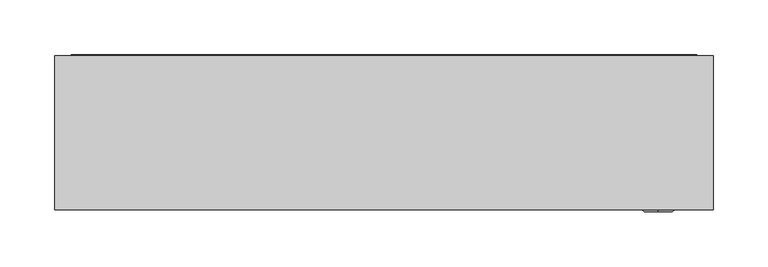
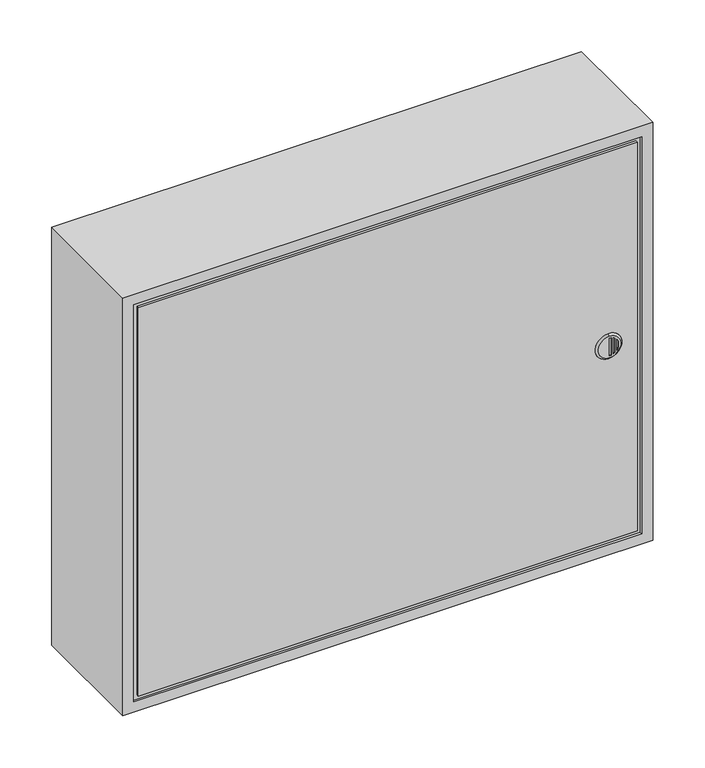
"""IFC4 building model written with IfcOpenShell, lengths in millimetres: proxy geometry, Unterverteiler : groß AP (120 PLE)."""

import ifcopenshell
import ifcopenshell.guid

model = None  # the IFC model being written
_history = None  # IfcOwnerHistory: only IFC2X3 demands one
_inside = {}  # id of a spatial element -> (the spatial element, [elements in it])
_under = {}  # id of a project, library or spatial element -> (it, [spatial elements below it])
_declared = {}  # id of a project -> (the project, [libraries it declares])
_typed = {}  # id of a type object -> (the type object, [elements of that type])
_made_of = {}  # id of a material, layer set ... -> (it, [elements and type objects made of it])


def new_model(schema):
    """Start an empty IFC model of exactly this schema.

    Asked for "IFC4X3", IfcOpenShell would pick the latest addendum, in which some entities
    have other attributes; the version numbers below select the first issue.
    IFC2X3 requires an IfcOwnerHistory on every rooted entity: one is made here for all.
    """
    global model, _history
    if schema == "IFC4X3":
        model = ifcopenshell.file(schema_version=(4, 3, 0, 0))
    else:
        model = ifcopenshell.file(schema=schema)
    _inside.clear()
    _under.clear()
    _declared.clear()
    _typed.clear()
    _made_of.clear()
    _history = None
    if model.schema == "IFC2X3":
        org = make("IfcOrganization", Name="unknown")
        user = make(
            "IfcPersonAndOrganization",
            ThePerson=make("IfcPerson", FamilyName="unknown"),
            TheOrganization=org,
        )
        app = make(
            "IfcApplication",
            ApplicationDeveloper=org,
            Version="unknown",
            ApplicationFullName="unknown",
            ApplicationIdentifier="unknown",
        )
        _history = make(
            "IfcOwnerHistory",
            OwningUser=user,
            OwningApplication=app,
            ChangeAction="ADDED",
            CreationDate=0,
        )
    return model


def make(cls, **values):
    """One entity of the class cls with the attributes given. An attribute that is None is left unset."""
    return model.create_entity(
        cls, **{name: value for name, value in values.items() if value is not None}
    )


def rooted(cls, **values):
    """An entity with a GlobalId (a new one), such as an element, a storey or a relation."""
    return make(cls, GlobalId=ifcopenshell.guid.new(), OwnerHistory=_history, **values)


def si_unit(unit_type, name, prefix=None):
    """IfcSIUnit, for example si_unit("LENGTHUNIT", "METRE", prefix="MILLI")."""
    return make("IfcSIUnit", UnitType=unit_type, Prefix=prefix, Name=name)


def assignment(units):
    """IfcUnitAssignment: the units of a project."""
    return None if units is None else make("IfcUnitAssignment", Units=units)


def point(xyz):
    """IfcCartesianPoint."""
    return None if xyz is None else make("IfcCartesianPoint", Coordinates=xyz)


def direction(xyz):
    """IfcDirection."""
    return None if xyz is None else make("IfcDirection", DirectionRatios=xyz)


def frame(location, z_axis=None, x_axis=None):
    """IfcAxis2Placement3D, a coordinate frame: its origin and axes. An axis left out is left unset."""
    return make(
        "IfcAxis2Placement3D",
        Location=point(location),
        Axis=direction(z_axis),
        RefDirection=direction(x_axis),
    )


def origin():
    """The frame at (0, 0, 0) with its axes left unset."""
    return frame((0.0, 0.0, 0.0))


def place(relative_to, where):
    """IfcLocalPlacement: puts the frame where relative to a parent placement (None: the world)."""
    return make(
        "IfcLocalPlacement", PlacementRelTo=relative_to, RelativePlacement=where
    )


def context(
    kind, dimensions, precision=None, world=None, true_north=None, identifier=None
):
    """IfcGeometricRepresentationContext, for example the 3D "Model" context."""
    return make(
        "IfcGeometricRepresentationContext",
        ContextIdentifier=identifier,
        ContextType=kind,
        CoordinateSpaceDimension=dimensions,
        Precision=precision,
        WorldCoordinateSystem=world,
        TrueNorth=true_north,
    )


def project(units=None, contexts=None):
    """IfcProject with its units and contexts."""
    return rooted(
        "IfcProject",
        Name="project",
        RepresentationContexts=contexts,
        UnitsInContext=assignment(units),
    )


def spatial(cls, under=None, at=None, **own):
    """A site, building, storey or space (cls), placed at a placement, below another one or the project."""
    s = rooted(cls, ObjectPlacement=at, **own)
    if under is not None:
        _under.setdefault(under.id(), (under, []))[1].append(s)
    return s


def polyline(points):
    """IfcPolyline through the points."""
    return make("IfcPolyline", Points=[point(p) for p in points])


def circle_curve(where, radius):
    """IfcCircle in the frame where."""
    return make("IfcCircle", Position=where, Radius=radius)


def outline(outer, holes=None, kind="AREA"):
    """IfcArbitraryClosedProfileDef: a profile drawn as a closed curve; with holes, ...WithVoids."""
    if holes is None:
        return make("IfcArbitraryClosedProfileDef", ProfileType=kind, OuterCurve=outer)
    return make(
        "IfcArbitraryProfileDefWithVoids",
        ProfileType=kind,
        OuterCurve=outer,
        InnerCurves=holes,
    )


def extrude(swept, where, along, depth):
    """IfcExtrudedAreaSolid: the profile swept, set in the frame where, extruded along a direction by depth."""
    return make(
        "IfcExtrudedAreaSolid",
        SweptArea=swept,
        Position=where,
        ExtrudedDirection=direction(along),
        Depth=depth,
    )


def shape(context_of_items, identifier, shape_type, items):
    """IfcShapeRepresentation: the items that make up one representation, for example the "Body"."""
    return make(
        "IfcShapeRepresentation",
        ContextOfItems=context_of_items,
        RepresentationIdentifier=identifier,
        RepresentationType=shape_type,
        Items=items,
    )


def source(mapping_origin, context_of_items, identifier, shape_type, items):
    """IfcRepresentationMap: a shape defined once, which mapped items show again and again."""
    return make(
        "IfcRepresentationMap",
        MappingOrigin=mapping_origin,
        MappedRepresentation=shape(context_of_items, identifier, shape_type, items),
    )


def transform(
    local_origin,
    x_axis=None,
    y_axis=None,
    z_axis=None,
    scale=None,
    scale2=None,
    scale3=None,
    uniform=True,
):
    """IfcCartesianTransformationOperator3D, or its non-uniform kind. x_axis, y_axis, z_axis: its Axis1, 2, 3."""
    if uniform:
        return make(
            "IfcCartesianTransformationOperator3D",
            Axis1=direction(x_axis),
            Axis2=direction(y_axis),
            LocalOrigin=point(local_origin),
            Scale=scale,
            Axis3=direction(z_axis),
        )
    return make(
        "IfcCartesianTransformationOperator3DnonUniform",
        Axis1=direction(x_axis),
        Axis2=direction(y_axis),
        LocalOrigin=point(local_origin),
        Scale=scale,
        Axis3=direction(z_axis),
        Scale2=scale2,
        Scale3=scale3,
    )


def mapped(mapping_source, mapping_target):
    """IfcMappedItem: shows the shape of a source again, moved by a transform."""
    return make(
        "IfcMappedItem", MappingSource=mapping_source, MappingTarget=mapping_target
    )


def made_of(thing, what):
    """Note that an element or type object is made of a material, layer set ...; save() writes the relation."""
    if what is not None:
        _made_of.setdefault(what.id(), (what, []))[1].append(thing)
    return thing


def element(
    cls,
    number,
    at=None,
    inside=None,
    cuts=None,
    type_object=None,
    material=None,
    context=None,
    identifier="Body",
    shape_type=None,
    held_by="IfcProductDefinitionShape",
    body=None,
    shapes=None,
    **own,
):
    """One element of the class cls, such as IfcWall. Its Tag is "e" and its number.

    at: its placement. inside: the storey or other place that contains it. cuts: it is an
    opening in that element (IfcRelVoidsElement). A single representation is given by context,
    identifier, shape_type and body (its items); several are given by shapes. held_by: the class
    of the entity that holds the representations. save() writes the other relations.
    """
    e = rooted(cls, Tag="e%d" % number, ObjectPlacement=at, **own)
    if body is not None:
        shapes = [shape(context, identifier, shape_type, body)]
    if shapes is not None:
        e.Representation = make(held_by, Representations=shapes)
    if inside is not None:
        _inside.setdefault(inside.id(), (inside, []))[1].append(e)
    if cuts is not None:
        rooted(
            "IfcRelVoidsElement", RelatingBuildingElement=cuts, RelatedOpeningElement=e
        )
    if type_object is not None:
        _typed.setdefault(type_object.id(), (type_object, []))[1].append(e)
    return made_of(e, material)


def aggregate(whole, parts):
    """IfcRelAggregates: a whole, such as a stair, and the parts it consists of."""
    return rooted("IfcRelAggregates", RelatingObject=whole, RelatedObjects=parts)


def save(model, path):
    """Write the relations noted so far, then the file.

    IfcRelAggregates (storeys below a building ...), IfcRelContainedInSpatialStructure (elements
    in a storey), IfcRelDefinesByType, IfcRelAssociatesMaterial and IfcRelDeclares: one each for
    every whole, place, type object, material and project.
    """
    for whole, parts in _under.values():
        aggregate(whole, parts)
    for where, things in _inside.values():
        rooted(
            "IfcRelContainedInSpatialStructure",
            RelatedElements=things,
            RelatingStructure=where,
        )
    for kind, things in _typed.values():
        rooted("IfcRelDefinesByType", RelatedObjects=things, RelatingType=kind)
    for what, things in _made_of.values():
        rooted("IfcRelAssociatesMaterial", RelatedObjects=things, RelatingMaterial=what)
    for by, libraries in _declared.values():
        rooted("IfcRelDeclares", RelatingContext=by, RelatedDefinitions=libraries)
    model.write(path)


def plane_surface(at):
    """IfcPlane: the flat surface through the origin of the frame at, square to its z axis."""
    return make("IfcPlane", Position=at)


def revolved_surface(curve, axis_point, axis_direction):
    """IfcSurfaceOfRevolution: the curve turned about the line through axis_point along axis_direction."""
    return make(
        "IfcSurfaceOfRevolution",
        SweptCurve=make("IfcArbitraryOpenProfileDef", ProfileType="CURVE", Curve=curve),
        AxisPosition=make("IfcAxis1Placement", Location=point(axis_point), Axis=direction(axis_direction)),
    )


def advanced_brep(points, edges, surfaces, faces):
    """IfcAdvancedBrep: a solid bounded by faces that lie on surfaces and meet in shared edges.

    An edge is (start, end): straight between two places in points (the first is 0);
    or (start, end, curve); or (start, end, curve, False) where it runs against its curve.
    A face is (place in surfaces, loops), or (place, loops, False) where it looks against
    its surface's normal. A loop lists edges by number (the first is 1), with a minus sign
    where the edge is run from its end to its start. The first loop is the outer one.
    """
    corners = [point(p) for p in points]
    vertices = [make("IfcVertexPoint", VertexGeometry=c) for c in corners]
    made = []
    for start, end, *more in edges:
        made.append(
            make(
                "IfcEdgeCurve",
                EdgeStart=vertices[start],
                EdgeEnd=vertices[end],
                EdgeGeometry=more[0] if more else make("IfcPolyline", Points=[corners[start], corners[end]]),
                SameSense=more[1] if len(more) > 1 else True,
            )
        )
    hull = []
    for where, loops, *sense in faces:
        bounds = []
        for j, loop in enumerate(loops):
            ring = [make("IfcOrientedEdge", EdgeElement=made[abs(k) - 1], Orientation=k > 0) for k in loop]
            bounds.append(
                make(
                    "IfcFaceOuterBound" if j == 0 else "IfcFaceBound",
                    Bound=make("IfcEdgeLoop", EdgeList=ring),
                    Orientation=True,
                )
            )
        hull.append(make("IfcAdvancedFace", Bounds=bounds, FaceSurface=surfaces[where], SameSense=sense[0] if sense else True))
    return make("IfcAdvancedBrep", Outer=make("IfcClosedShell", CfsFaces=hull))


def electrical_equipment_9f8c9aa4(model_context):
    return source(origin(), model_context, "Body", "SolidModel", [
        extrude(outline(polyline([(285.0, 0.0), (-285.0, 0.0), (-285.0, 1.0), (285.0, 1.0), (285.0, 0.0)])), frame((0.0, 0.0, 1215.0), z_axis=(0.0, 0.0, 1.0), x_axis=(1.0, 0.0, 0.0)), (0.0, 0.0, 1.0), 470.0),
        advanced_brep(
        [(300.0, -140.0, 1700.0), (-300.0, -140.0, 1700.0), (-300.0, -140.0, 1200.0), (300.0, -140.0, 1200.0), (287.5084747, -140.0, 1687.5084747), (287.5084747, -140.0, 1212.4915253), (-287.5084747, -140.0, 1212.4915253), (-287.5084747, -140.0, 1687.5084747), (282.5084747, -140.0, 1217.4915253), (282.5084747, -140.0, 1682.5084747), (-282.5084747, -140.0, 1682.5084747), (-282.5084747, -140.0, 1217.4915253), (250.0, -140.0, 1465.0), (250.0, -140.0, 1435.0), (300.0, 0.0, 1700.0), (300.0, 0.0, 1200.0), (-300.0, 0.0, 1200.0), (-300.0, 0.0, 1700.0), (287.5084747, -137.5412427, 1687.5084747), (287.5084747, -137.5412427, 1212.4915253), (282.5084747, -137.5412427, 1217.4915253), (282.5084747, -137.5412427, 1682.5084747), (-287.5084747, -137.5412427, 1212.4915253), (-282.5084747, -137.5412427, 1217.4915253), (-287.5084747, -137.5412427, 1687.5084747), (-282.5084747, -137.5412427, 1682.5084747), (250.0, -141.0, 1439.5419588), (252.0, -141.0, 1439.7341948), (252.0, -141.0, 1460.3497229), (250.0, -141.0, 1460.5419588), (254.0, -141.0, 1440.3337149), (256.0, -141.0, 1441.4251148), (256.0, -141.0, 1458.6588028), (254.0, -141.0, 1459.7502027), (258.0, -141.0, 1443.2412236), (260.0, -141.0, 1446.8403967), (260.0, -141.0, 1453.2435209), (258.0, -141.0, 1456.8426941), (250.0, -142.0, 1439.5419588), (252.0, -142.0, 1439.7341948), (252.0, -142.0, 1460.3497229), (250.0, -142.0, 1460.5419588), (254.0, -142.0, 1440.3337149), (256.0, -142.0, 1441.4251148), (256.0, -142.0, 1458.6588028), (254.0, -142.0, 1459.7502027), (258.0, -142.0, 1443.2412236), (260.0, -142.0, 1446.8403967), (260.0, -142.0, 1453.2435209), (258.0, -142.0, 1456.8426941), (250.0, -142.0, 1437.25), (250.0, -142.0, 1462.75)],
        [
            (0, 1),
            (1, 2),
            (2, 3),
            (3, 0),
            (4, 5),
            (5, 6),
            (6, 7),
            (7, 4),
            (8, 9),
            (9, 10),
            (10, 11),
            (11, 8),
            (12, 13, circle_curve(frame((250.0, -140.0, 1450.0), z_axis=(0.0, 1.0, 0.0), x_axis=(0.0, 0.0, -1.0)), 15.0)),
            (13, 12, circle_curve(frame((250.0, -140.0, 1450.0), z_axis=(0.0, 1.0, 0.0), x_axis=(0.0, 0.0, 1.0)), 15.0)),
            (14, 15),
            (15, 16),
            (16, 17),
            (17, 14),
            (0, 14),
            (17, 1),
            (16, 2),
            (15, 3),
            (18, 19),
            (19, 5),
            (4, 18),
            (8, 20),
            (20, 21),
            (21, 9),
            (19, 22),
            (22, 6),
            (11, 23),
            (23, 20),
            (22, 24),
            (24, 7),
            (10, 25),
            (25, 23),
            (24, 18),
            (25, 21),
            (26, 27, circle_curve(frame((250.0, -141.0, 1450.0419588), z_axis=(0.0, -1.0, 0.0), x_axis=(0.0, 0.0, 1.0)), 10.5)),
            (27, 28),
            (28, 29, circle_curve(frame((250.0, -141.0, 1450.0419588), z_axis=(0.0, -1.0, 0.0), x_axis=(0.0, 0.0, 1.0)), 10.5)),
            (29, 26),
            (30, 31, circle_curve(frame((250.0, -141.0, 1450.0419588), z_axis=(0.0, -1.0, 0.0), x_axis=(0.0, 0.0, 1.0)), 10.5)),
            (31, 32),
            (32, 33, circle_curve(frame((250.0, -141.0, 1450.0419588), z_axis=(0.0, -1.0, 0.0), x_axis=(0.0, 0.0, 1.0)), 10.5)),
            (33, 30),
            (34, 35, circle_curve(frame((250.0, -141.0, 1450.0419588), z_axis=(0.0, -1.0, 0.0), x_axis=(0.0, 0.0, 1.0)), 10.5)),
            (35, 36),
            (36, 37, circle_curve(frame((250.0, -141.0, 1450.0419588), z_axis=(0.0, -1.0, 0.0), x_axis=(0.0, 0.0, 1.0)), 10.5)),
            (37, 34),
            (26, 38),
            (38, 39, circle_curve(frame((250.0, -142.0, 1450.0419588), z_axis=(0.0, -1.0, 0.0), x_axis=(0.0, 0.0, 1.0)), 10.5)),
            (39, 27),
            (39, 40),
            (40, 28),
            (40, 41, circle_curve(frame((250.0, -142.0, 1450.0419588), z_axis=(0.0, -1.0, 0.0), x_axis=(0.0, 0.0, 1.0)), 10.5)),
            (41, 29),
            (41, 38),
            (30, 42),
            (42, 43, circle_curve(frame((250.0, -142.0, 1450.0419588), z_axis=(0.0, -1.0, 0.0), x_axis=(0.0, 0.0, 1.0)), 10.5)),
            (43, 31),
            (43, 44),
            (44, 32),
            (44, 45, circle_curve(frame((250.0, -142.0, 1450.0419588), z_axis=(0.0, -1.0, 0.0), x_axis=(0.0, 0.0, 1.0)), 10.5)),
            (45, 33),
            (45, 42),
            (34, 46),
            (46, 47, circle_curve(frame((250.0, -142.0, 1450.0419588), z_axis=(0.0, -1.0, 0.0), x_axis=(0.0, 0.0, 1.0)), 10.5)),
            (47, 35),
            (47, 48),
            (48, 36),
            (48, 49, circle_curve(frame((250.0, -142.0, 1450.0419588), z_axis=(0.0, -1.0, 0.0), x_axis=(0.0, 0.0, 1.0)), 10.5)),
            (49, 37),
            (49, 46),
            (50, 51, circle_curve(frame((250.0, -142.0, 1450.0), z_axis=(0.0, -1.0, 0.0), x_axis=(0.0, 0.0, -1.0)), 12.75)),
            (51, 50, circle_curve(frame((250.0, -142.0, 1450.0), z_axis=(0.0, -1.0, 0.0), x_axis=(0.0, 0.0, 1.0)), 12.75)),
            (50, 13),
            (12, 51),
        ],
        [
            plane_surface(frame((-300.0, -140.0, 1700.0), z_axis=(0.0, -1.0, 0.0), x_axis=(-1.0, 0.0, 0.0))),
            plane_surface(frame((-300.0, 0.0, 1700.0), z_axis=(0.0, 1.0, 0.0), x_axis=(1.0, 0.0, 0.0))),
            plane_surface(frame((300.0, -140.0, 1700.0), z_axis=(0.0, 0.0, 1.0), x_axis=(0.0, 1.0, 0.0))),
            plane_surface(frame((-300.0, -140.0, 1700.0), z_axis=(-1.0, 0.0, 0.0), x_axis=(0.0, 1.0, 0.0))),
            plane_surface(frame((-300.0, -140.0, 1200.0), z_axis=(0.0, 0.0, -1.0), x_axis=(0.0, 1.0, 0.0))),
            plane_surface(frame((300.0, -140.0, 1200.0), z_axis=(1.0, 0.0, 0.0), x_axis=(0.0, 1.0, 0.0))),
            plane_surface(frame((287.5084747, -140.0, 1687.5084747), z_axis=(-1.0, 0.0, 0.0), x_axis=(0.0, 0.0, -1.0))),
            plane_surface(frame((282.5084747, -137.5412427, 1682.5084747), z_axis=(1.0, 0.0, 0.0), x_axis=(0.0, 0.0, -1.0))),
            plane_surface(frame((287.5084747, -140.0, 1212.4915253), z_axis=(0.0, 0.0, 1.0), x_axis=(-1.0, 0.0, 0.0))),
            plane_surface(frame((282.5084747, -137.5412427, 1217.4915253), z_axis=(0.0, 0.0, -1.0), x_axis=(-1.0, 0.0, 0.0))),
            plane_surface(frame((-287.5084747, -140.0, 1212.4915253), z_axis=(1.0, 0.0, 0.0), x_axis=(0.0, 0.0, 1.0))),
            plane_surface(frame((-282.5084747, -137.5412427, 1217.4915253), z_axis=(-1.0, 0.0, 0.0), x_axis=(0.0, 0.0, 1.0))),
            plane_surface(frame((-287.5084747, -140.0, 1687.5084747), z_axis=(0.0, 0.0, -1.0), x_axis=(1.0, 0.0, 0.0))),
            plane_surface(frame((-287.5084747, -137.5412427, 1687.5084747), z_axis=(0.0, -1.0, 0.0), x_axis=(1.0, 0.0, 0.0))),
            plane_surface(frame((-282.5084747, -137.5412427, 1682.5084747), z_axis=(0.0, 0.0, 1.0), x_axis=(1.0, 0.0, 0.0))),
            plane_surface(frame((250.0, -141.0, 1460.5419588), z_axis=(0.0, -1.0, 0.0), x_axis=(0.0, 0.0, 1.0))),
            revolved_surface(polyline([(250.0, -141.0, 1460.5419588), (250.0, -142.0, 1460.5419588)]), (250.0, -142.0, 1450.0419588), (0.0, 1.0, 0.0)),
            plane_surface(frame((252.0, -141.0, 1460.3497229), z_axis=(-1.0, 0.0, 0.0), x_axis=(0.0, -1.0, 0.0))),
            plane_surface(frame((250.0, -141.0, 1439.5419588), z_axis=(1.0, 0.0, 0.0), x_axis=(0.0, -1.0, 0.0))),
            plane_surface(frame((256.0, -141.0, 1458.6588028), z_axis=(-1.0, 0.0, 0.0), x_axis=(0.0, -1.0, 0.0))),
            plane_surface(frame((254.0, -141.0, 1440.3337149), z_axis=(1.0, 0.0, 0.0), x_axis=(0.0, -1.0, 0.0))),
            plane_surface(frame((260.0, -141.0, 1453.2435209), z_axis=(-1.0, 0.0, 0.0), x_axis=(0.0, -1.0, 0.0))),
            plane_surface(frame((258.0, -141.0, 1443.2412236), z_axis=(1.0, 0.0, 0.0), x_axis=(0.0, -1.0, 0.0))),
            plane_surface(frame((250.0, -142.0, 1450.0), z_axis=(0.0, -1.0, 0.0), x_axis=(-1.0, 0.0, 0.0))),
            revolved_surface(polyline([(250.0, -142.0, 1437.250000005625), (250.0, -140.0, 1435.0)]), (250.0, -153.3333333, 1450.0), (0.0, 1.0, 0.0)),
            revolved_surface(polyline([(250.0, -142.0, 1462.749999994375), (250.0, -140.0, 1465.0)]), (250.0, -153.3333333, 1450.0), (0.0, 1.0, 0.0)),
        ],
        [
            (0, [[1, 2, 3, 4], [5, 6, 7, 8]]),
            (0, [[9, 10, 11, 12], [13, 14]]),
            (1, [[15, 16, 17, 18]]),
            (2, [[-1, 19, -18, 20]]),
            (3, [[-2, -20, -17, 21]]),
            (4, [[-3, -21, -16, 22]]),
            (5, [[-4, -22, -15, -19]]),
            (6, [[23, 24, -5, 25]]),
            (7, [[26, 27, 28, -9]]),
            (8, [[-24, 29, 30, -6]]),
            (9, [[-26, -12, 31, 32]]),
            (10, [[-30, 33, 34, -7]]),
            (11, [[-31, -11, 35, 36]]),
            (12, [[-25, -8, -34, 37]]),
            (13, [[-23, -37, -33, -29], [-27, -32, -36, 38]]),
            (14, [[-28, -38, -35, -10]]),
            (15, [[39, 40, 41, 42]]),
            (15, [[43, 44, 45, 46]]),
            (15, [[47, 48, 49, 50]]),
            (16, [[-39, 51, 52, 53]]),
            (17, [[-40, -53, 54, 55]]),
            (16, [[-41, -55, 56, 57]]),
            (18, [[-42, -57, 58, -51]]),
            (16, [[-43, 59, 60, 61]]),
            (19, [[-44, -61, 62, 63]]),
            (16, [[-45, -63, 64, 65]]),
            (20, [[-46, -65, 66, -59]]),
            (16, [[-47, 67, 68, 69]]),
            (21, [[-48, -69, 70, 71]]),
            (16, [[-49, -71, 72, 73]]),
            (22, [[-50, -73, 74, -67]]),
            (23, [[75, 76], [-52, -58, -56, -54], [-60, -66, -64, -62], [-68, -74, -72, -70]]),
            (24, [[-75, 77, -13, 78]]),
            (25, [[-76, -78, -14, -77]]),
        ],
    ),
    ])


if __name__ == "__main__":
    model = new_model("IFC4")
    model_context = context("Model", 3, world=origin())
    ifc_project = project(units=[si_unit("LENGTHUNIT", "METRE", prefix="MILLI")], contexts=[model_context])
    site = spatial("IfcSite", under=ifc_project)
    building = spatial("IfcBuilding", under=site)
    placement = place(None, origin())
    electrical_equipment_shape = electrical_equipment_9f8c9aa4(model_context)
    element("IfcBuildingElementProxy", 1, Name="Unterverteiler : groß AP (120 PLE)", ObjectType="Unterverteiler : groß AP (120 PLE)", at=placement, inside=building, context=model_context, shape_type="MappedRepresentation", body=[
        mapped(electrical_equipment_shape, transform((0.0, 0.0, 0.0), x_axis=(1.0, 0.0, 0.0), y_axis=(0.0, 1.0, 0.0), z_axis=(0.0, 0.0, 1.0))),
    ])
    save(model, "model.ifc")

# Revit data of these elements
# Type "Unterverteiler : groß AP (120 PLE)"
#   Kostengruppe = "444"
#   DIN 276 = "Starkstrom"
#   Tiefe UP = 0.001 m
#   Länge Symbol = 0.001 m
#   Tiefe AP = 0.140 m
#   Leistungsfaktor = 1
#   Installationshöhe [instance default] = 1.200 m
#   Höhe Kabelkanalanschluss [instance default] = 0.060 m
#   Höhe = 0.500 m
#   built-in parameter 1140140 [instance default] = 1 (stored number, unit not read)
#   Durchmesser Leerrohranschluss 02 [instance default] = 0.050 m
#   Durchmesser Leerrohranschluss 01 [instance default] = 0.050 m
#   Breite Kabelkanalanschluss [instance default] = 0.150 m
#   Breite = 0.600 m
#   UP = no
#   built-in parameter 1140142 [instance default] = -1
#   built-in parameter 1155100 [instance default] = -1
#   AP = yes
#   Oberfläche [instance default] = none
#   Lastklassifizierung = Energie
#   Default Elevation = 0
